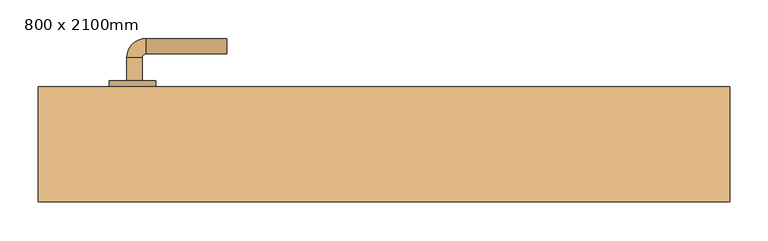
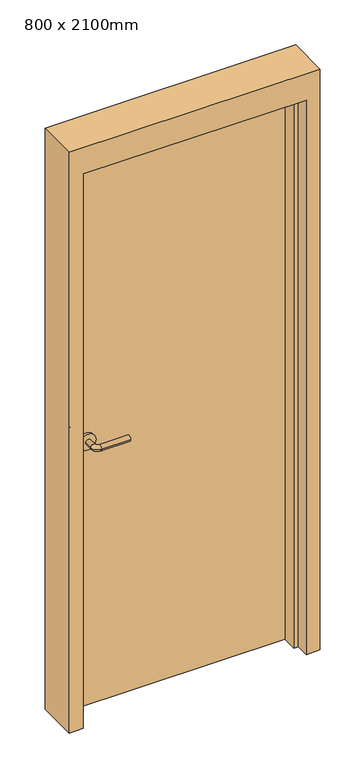
"""IFC4 building model written with IfcOpenShell, lengths in millimetres: door geometry, M_Puerta-De_paso-Simple-Paneles_planos : 800 x 2100mm."""

from ifc_helpers import new_model, si_unit, point, frame, frame_2d, origin, origin_with_axes, place, context, project, spatial, polyline, circle_curve, ellipse_curve, trimmed, segment, composite_curve, outline, extrude, faceted_brep, source, transform, mapped, element, save
from ifc_brep_helpers import plane_surface, cylinder_surface, revolved_surface, advanced_brep


def door_800_x_2100mm_2fbfaaac(model_context):
    return source(origin(), model_context, "Body", "SolidModel", [
        advanced_brep(
        [(-334.990625, 3.35, 1000.0), (-314.990625, 3.35, 1000.0), (-314.990625, -26.65, 1000.0), (-334.990625, -26.65, 1000.0), (-309.990625, -31.65, 1000.0), (-309.990625, -51.65, 1000.0), (-204.990625, -51.65, 1000.0), (-204.990625, -31.65, 1000.0)],
        [
            (0, 1, circle_curve(frame((-324.990625, 3.35, 1000.0), z_axis=(0.0, 1.0, 0.0), x_axis=(1.0, 0.0, 0.0)), 10.0)),
            (1, 0, circle_curve(frame((-324.990625, 3.35, 1000.0), z_axis=(0.0, 1.0, 0.0), x_axis=(1.0, 0.0, 0.0)), 10.0)),
            (1, 2),
            (2, 3, circle_curve(frame((-324.990625, -26.65, 1000.0), z_axis=(0.0, 1.0, 0.0), x_axis=(1.0, 0.0, 0.0)), 10.0)),
            (3, 0),
            (3, 2, circle_curve(frame((-324.990625, -26.65, 1000.0), z_axis=(0.0, 1.0, 0.0), x_axis=(1.0, 0.0, 0.0)), 10.0)),
            (4, 5, circle_curve(frame((-309.990625, -41.65, 1000.0), z_axis=(-1.0, 0.0, 0.0), x_axis=(0.0, 1.0, 0.0)), 10.0)),
            (5, 3, circle_curve(frame((-309.990625, -26.65, 1000.0), z_axis=(0.0, 0.0, -1.0), x_axis=(-1.0, 0.0, 0.0)), 25.0)),
            (2, 4, circle_curve(frame((-309.990625, -26.65, 1000.0), z_axis=(0.0, 0.0, 1.0), x_axis=(-1.0, 0.0, 0.0)), 5.0)),
            (5, 4, circle_curve(frame((-309.990625, -41.65, 1000.0), z_axis=(-1.0, 0.0, 0.0), x_axis=(0.0, 1.0, 0.0)), 10.0)),
            (6, 7, circle_curve(frame((-204.990625, -41.65, 1000.0), z_axis=(1.0, 0.0, 0.0), x_axis=(0.0, 1.0, 0.0)), 10.0)),
            (7, 6, circle_curve(frame((-204.990625, -41.65, 1000.0), z_axis=(1.0, 0.0, 0.0), x_axis=(0.0, 1.0, 0.0)), 10.0)),
            (4, 7),
            (6, 5),
        ],
        [
            plane_surface(frame((-324.990625, 3.35, 1000.0), z_axis=(0.0, 1.0, 0.0), x_axis=(0.0, 0.0, 1.0))),
            cylinder_surface(frame((-324.990625, 3.35, 1000.0), z_axis=(0.0, 1.0, 0.0), x_axis=(1.0, 0.0, 0.0)), 10.0),
            revolved_surface(trimmed(ellipse_curve(frame((-324.990625, -26.65, 1000.0), z_axis=(0.0, -1.0, 0.0), x_axis=(1.0, 0.0, 0.0)), 10.0, 10.0), [point((-334.990625, -26.65, 1000.0))], [point((-314.990625, -26.65, 1000.0))], True, "CARTESIAN"), (-309.990625, -26.65, 1000.0), (0.0, 0.0, -1.0)),
            revolved_surface(trimmed(ellipse_curve(frame((-324.990625, -26.65, 1000.0), z_axis=(0.0, -1.0, 0.0), x_axis=(1.0, 0.0, 0.0)), 10.0, 10.0), [point((-314.990625, -26.65, 1000.0))], [point((-334.990625, -26.65, 1000.0))], True, "CARTESIAN"), (-309.990625, -26.65, 1000.0), (0.0, 0.0, -1.0)),
            plane_surface(frame((-204.990625, -41.65, 1000.0), z_axis=(1.0, 0.0, 0.0), x_axis=(0.0, 0.0, 1.0))),
            cylinder_surface(frame((-309.990625, -41.65, 1000.0), z_axis=(-1.0, 0.0, 0.0), x_axis=(0.0, 1.0, 0.0)), 10.0),
        ],
        [
            (0, [[1, 2]]),
            (1, [[3, 4, 5, -2]]),
            (1, [[-5, 6, -3, -1]]),
            (2, [[7, 8, -4, 9]]),
            (3, [[10, -9, -6, -8]]),
            (4, [[11, 12]]),
            (5, [[13, -11, 14, -7]]),
            (5, [[-14, -12, -13, -10]]),
        ],
    ),
        extrude(outline(composite_curve([segment(trimmed(circle_curve(frame_2d((1000.0, -327.490625)), 30.0), [point((1000.0, -357.490625))], [point((1000.0, -297.490625))], False, "CARTESIAN"), True, "CONTINUOUS"), segment(trimmed(circle_curve(frame_2d((1000.0, -327.490625)), 30.0), [point((1000.0, -297.490625))], [point((1000.0, -357.490625))], False, "CARTESIAN"), True, "CONTINUOUS")], self_intersect=False)), frame((0.0, 3.35, 0.0), z_axis=(0.0, 1.0, 0.0), x_axis=(0.0, 0.0, 1.0)), (0.0, 0.0, 1.0), 8.0),
        advanced_brep(
        [(-334.990625, 64.35, 1000.0), (-314.990625, 64.35, 1000.0), (-334.990625, 94.35, 1000.0), (-314.990625, 94.35, 1000.0), (-309.990625, 99.35, 1000.0), (-309.990625, 119.35, 1000.0), (-204.990625, 119.35, 1000.0), (-204.990625, 99.35, 1000.0)],
        [
            (0, 1, circle_curve(frame((-324.990625, 64.35, 1000.0), z_axis=(0.0, -1.0, 0.0), x_axis=(1.0, 0.0, 0.0)), 10.0)),
            (1, 0, circle_curve(frame((-324.990625, 64.35, 1000.0), z_axis=(0.0, -1.0, 0.0), x_axis=(1.0, 0.0, 0.0)), 10.0)),
            (0, 2),
            (2, 3, circle_curve(frame((-324.990625, 94.35, 1000.0), z_axis=(0.0, -1.0, 0.0), x_axis=(1.0, 0.0, 0.0)), 10.0)),
            (3, 1),
            (3, 2, circle_curve(frame((-324.990625, 94.35, 1000.0), z_axis=(0.0, -1.0, 0.0), x_axis=(1.0, 0.0, 0.0)), 10.0)),
            (4, 3, circle_curve(frame((-309.990625, 94.35, 1000.0), z_axis=(0.0, 0.0, 1.0), x_axis=(-1.0, 0.0, 0.0)), 5.0)),
            (2, 5, circle_curve(frame((-309.990625, 94.35, 1000.0), z_axis=(0.0, 0.0, -1.0), x_axis=(-1.0, 0.0, 0.0)), 25.0)),
            (5, 4, circle_curve(frame((-309.990625, 109.35, 1000.0), z_axis=(-1.0, 0.0, 0.0), x_axis=(0.0, -1.0, 0.0)), 10.0)),
            (4, 5, circle_curve(frame((-309.990625, 109.35, 1000.0), z_axis=(-1.0, 0.0, 0.0), x_axis=(0.0, -1.0, 0.0)), 10.0)),
            (6, 7, circle_curve(frame((-204.990625, 109.35, 1000.0), z_axis=(1.0, 0.0, 0.0), x_axis=(0.0, -1.0, 0.0)), 10.0)),
            (7, 6, circle_curve(frame((-204.990625, 109.35, 1000.0), z_axis=(1.0, 0.0, 0.0), x_axis=(0.0, -1.0, 0.0)), 10.0)),
            (5, 6),
            (7, 4),
        ],
        [
            plane_surface(frame((-324.990625, 64.35, 1000.0), z_axis=(0.0, -1.0, 0.0), x_axis=(0.0, 0.0, 1.0))),
            cylinder_surface(frame((-324.990625, 64.35, 1000.0), z_axis=(0.0, -1.0, 0.0), x_axis=(1.0, 0.0, 0.0)), 10.0),
            revolved_surface(trimmed(ellipse_curve(frame((-324.990625, 94.35, 1000.0), z_axis=(0.0, -1.0, 0.0), x_axis=(1.0, 0.0, 0.0)), 10.0, 10.0), [point((-334.990625, 94.35, 1000.0))], [point((-314.990625, 94.35, 1000.0))], True, "CARTESIAN"), (-309.990625, 94.35, 1000.0), (0.0, 0.0, -1.0)),
            revolved_surface(trimmed(ellipse_curve(frame((-324.990625, 94.35, 1000.0), z_axis=(0.0, -1.0, 0.0), x_axis=(1.0, 0.0, 0.0)), 10.0, 10.0), [point((-314.990625, 94.35, 1000.0))], [point((-334.990625, 94.35, 1000.0))], True, "CARTESIAN"), (-309.990625, 94.35, 1000.0), (0.0, 0.0, -1.0)),
            plane_surface(frame((-204.990625, 109.35, 1000.0), z_axis=(1.0, 0.0, 0.0), x_axis=(0.0, 0.0, 1.0))),
            cylinder_surface(frame((-309.990625, 109.35, 1000.0), z_axis=(-1.0, 0.0, 0.0), x_axis=(0.0, -1.0, 0.0)), 10.0),
        ],
        [
            (0, [[1, 2]]),
            (1, [[-1, 3, 4, 5]]),
            (1, [[-2, -5, 6, -3]]),
            (2, [[7, -4, 8, 9]]),
            (3, [[-8, -6, -7, 10]]),
            (4, [[11, 12]]),
            (5, [[-9, 13, -12, 14]]),
            (5, [[-10, -14, -11, -13]]),
        ],
    ),
        extrude(outline(composite_curve([segment(trimmed(circle_curve(frame_2d((1000.0, -327.490625)), 30.0), [point((1000.0, -357.490625))], [point((1000.0, -297.490625))], False, "CARTESIAN"), True, "CONTINUOUS"), segment(trimmed(circle_curve(frame_2d((1000.0, -327.490625)), 30.0), [point((1000.0, -297.490625))], [point((1000.0, -357.490625))], False, "CARTESIAN"), True, "CONTINUOUS")], self_intersect=False)), frame((0.0, 56.35, 0.0), z_axis=(0.0, 1.0, 0.0), x_axis=(0.0, 0.0, 1.0)), (0.0, 0.0, 1.0), 8.0),
        extrude(outline(polyline([(400.0, 11.35), (-400.0, 11.35), (-400.0, 56.35), (400.0, 56.35), (400.0, 11.35)])), origin_with_axes(), (0.0, 0.0, 1.0), 2100.0),
        faceted_brep([(400.0, 6.5875, 0.0), (400.0, 56.35, 0.0), (450.0, 56.35, 0.0), (450.0, -93.65, 0.0), (400.0, -93.65, 0.0), (400.0, -44.4375, 0.0), (384.125, -44.4375, 0.0), (384.125, 6.5875, 0.0), (400.0, 6.5875, 2100.0), (400.0, 56.35, 2100.0), (-400.0, 56.35, 2100.0), (-400.0, 56.35, 0.0), (-450.0, 56.35, 0.0), (-450.0, 56.35, 2200.0), (450.0, 56.35, 2200.0), (450.0, -93.65, 2200.0), (-450.0, -93.65, 2200.0), (-450.0, -93.65, 0.0), (-400.0, -93.65, 0.0), (-400.0, -93.65, 2100.0), (400.0, -93.65, 2100.0), (400.0, -44.4375, 2100.0), (-400.0, -44.4375, 2100.0), (-400.0, -44.4375, 0.0), (-384.125, -44.4375, 0.0), (-384.125, -44.4375, 2084.125), (384.125, -44.4375, 2084.125), (384.125, 6.5875, 2084.125), (-384.125, 6.5875, 2084.125), (-384.125, 6.5875, 0.0), (-400.0, 6.5875, 0.0), (-400.0, 6.5875, 2100.0)], [[[0, 1, 2, 3, 4, 5, 6, 7]], [[1, 0, 8, 9]], [[2, 1, 9, 10, 11, 12, 13, 14]], [[3, 2, 14, 15]], [[4, 3, 15, 16, 17, 18, 19, 20]], [[5, 4, 20, 21]], [[6, 5, 21, 22, 23, 24, 25, 26]], [[7, 6, 26, 27]], [[0, 7, 27, 28, 29, 30, 31, 8]], [[9, 8, 31, 10]], [[20, 19, 22, 21]], [[26, 25, 28, 27]], [[12, 11, 30, 29, 24, 23, 18, 17]], [[11, 10, 31, 30]], [[13, 12, 17, 16]], [[19, 18, 23, 22]], [[25, 24, 29, 28]], [[15, 14, 13, 16]]]),
    ])


if __name__ == "__main__":
    model = new_model("IFC4")
    model_context = context("Model", 3, world=origin())
    ifc_project = project(units=[si_unit("LENGTHUNIT", "METRE", prefix="MILLI")], contexts=[model_context])
    site = spatial("IfcSite", under=ifc_project)
    building = spatial("IfcBuilding", under=site)
    placement = place(None, origin())
    door_800_x_2100mm_shape = door_800_x_2100mm_2fbfaaac(model_context)
    element("IfcDoor", 1, ObjectType="M_Puerta-De_paso-Simple-Paneles_planos : 800 x 2100mm", at=placement, inside=building, context=model_context, shape_type="MappedRepresentation", body=[
        mapped(door_800_x_2100mm_shape, transform((0.0, 0.0, 0.0), x_axis=(1.0, 0.0, 0.0), y_axis=(0.0, 1.0, 0.0), z_axis=(0.0, 0.0, 1.0))),
    ])
    save(model, "model.ifc")

# Revit data of these elements
# Type "M_Puerta-De_paso-Simple-Paneles_planos : 800 x 2100mm"
#   Type Mark = "47"
#   Analytic Construction = "Madera"
#   Thickness = 0.045 m
#   Thermal Resistance (R) = 0.455703 (m²·K)/W
#   Ángulo de batiente [instance default] = 90.00°
#   Altura del pasador = 1.00 m
#   Rough Width [instance default] = 0.90 m
#   Rough Height [instance default] = 2.20 m
#   Altura de hueco MF [instance default] = 0.10 m
#   Anchura de hueco MF [instance default] = 0.10 m
#   Cálculo de la incrustación [instance default] = 0.105 m
#   Incrustación de albañilería [instance default] = 0.025 m
#   Height = 2.10 m
#   Width = 0.80 m
#   Heat Transfer Coefficient (U) = 2.19465 W/(m²·K)
#   Profundidad del marco del albañilería = 0.15 m
#   Marco del albañilería [instance default] = yes
#   Function = 1
#   Marco de muro seco [instance default] = no
#   Material de panel = Madera - Abedul
#   Material de estructura = Metal - Acabado de pintura - Gris
#   Material de tirador = Aluminio 1
#   Visual Light Transmittance = 0
#   Solar Heat Gain Coefficient = 0
#   Wall Closure = (empty or 0)
# Element 1 (IfcDoor, "M_Puerta-De_paso-Simple-Paneles_planos : 800 x 2100mm")
#   Materials on its faces: "Aluminio 1", "Metal - Acabado de pintura - Gris", "Madera - Abedul"
# Materials
#   "Madera - Abedul": class "Madera", colour RGB 173 132 96, transparency 0, Cost = 0
#   "Metal - Acabado de pintura - Gris": class "Pintura", colour RGB 178 178 178, transparency 0, Cost = 0
#   "Aluminio 1": class "Metal", colour RGB 244 245 246, transparency 0, Description = "Aluminio 6061", Cost = 0
